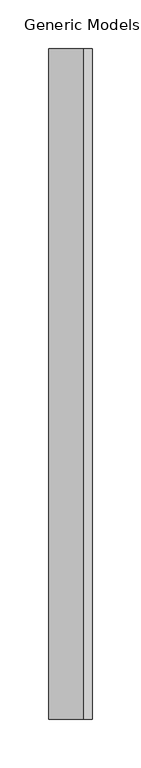
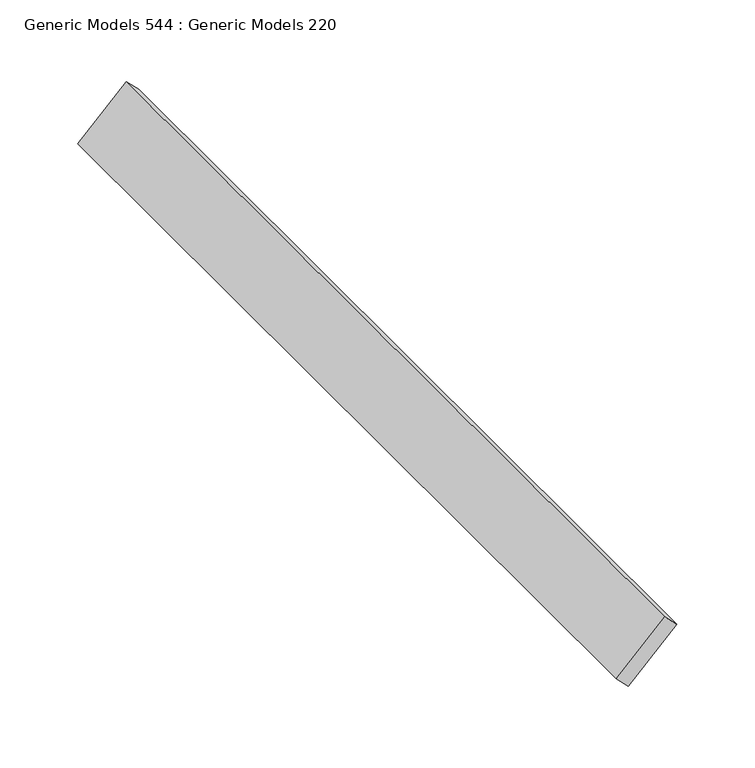
"""IFC4 building model written with IfcOpenShell, lengths in millimetres: proxy geometry, Generic Models 544 : Generic Models 220."""

from ifc_helpers import new_model, si_unit, frame, origin, place, context, project, spatial, polyline, outline, extrude, source, transform, mapped, element, save


def generic_models_544_generic_models_220_69997cfd(model_context):
    return source(origin(), model_context, "Body", "SweptSolid", [
        extrude(outline(polyline([(0.0, -12.7000001), (0.0, 0.0), (690.8142348, 0.0), (690.8142348, -12.7000001), (0.0, -12.7000001)])), frame((7841.3059863, 4539.4872686, 124874.6399101), z_axis=(0.7071067811868034, 0.0, 0.7071067811862918), x_axis=(0.0, -1.0, 0.0)), (0.0, 0.0, 1.0), 50.8),
    ])


if __name__ == "__main__":
    model = new_model("IFC4")
    model_context = context("Model", 3, world=origin())
    ifc_project = project(units=[si_unit("LENGTHUNIT", "METRE", prefix="MILLI")], contexts=[model_context])
    site = spatial("IfcSite", under=ifc_project)
    building = spatial("IfcBuilding", under=site)
    placement = place(None, origin())
    generic_models_544_generic_models_220_shape = generic_models_544_generic_models_220_69997cfd(model_context)
    element("IfcBuildingElementProxy", 1, Name="Generic Models 544 : Generic Models 220", ObjectType="Generic Models 544 : Generic Models 220", at=placement, inside=building, context=model_context, shape_type="MappedRepresentation", body=[
        mapped(generic_models_544_generic_models_220_shape, transform((0.0, 0.0, 0.0), x_axis=(1.0, 0.0, 0.0), y_axis=(0.0, 1.0, 0.0), z_axis=(0.0, 0.0, 1.0))),
    ])
    save(model, "model.ifc")

# Revit data of these elements
# Element 1 (IfcBuildingElementProxy, "Generic Models 544 : Generic Models 220")
#   Materials on its faces: "_WOOD TONE ALUMINUM EXTRUSION SLAT BY KNOTWOOD"
# Materials
#   "_WOOD TONE ALUMINUM EXTRUSION SLAT BY KNOTWOOD": class "Generic", colour RGB 177 130 114, transparency 0, Cost = 0
